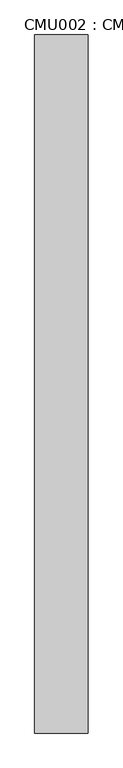
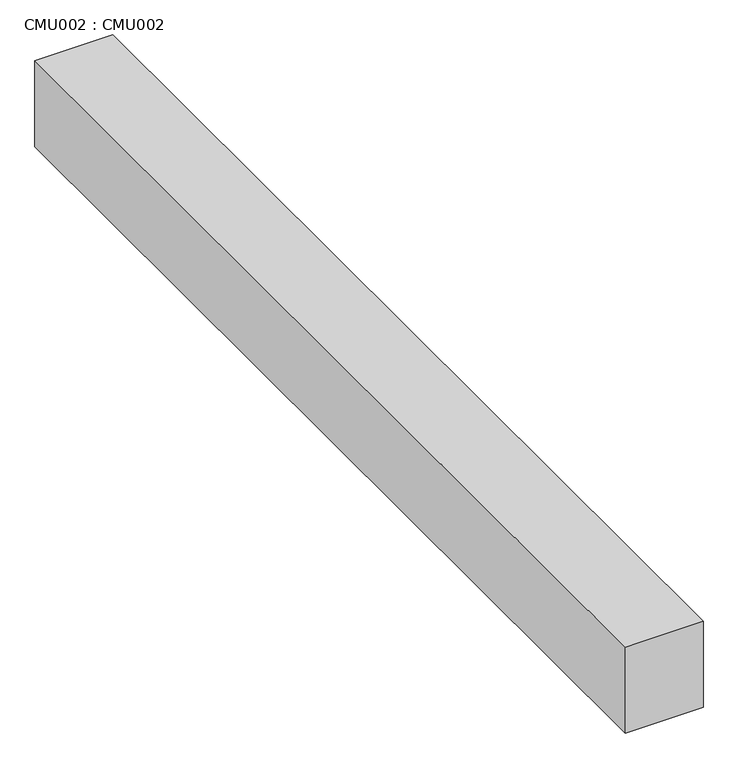
"""IFC4 building model written with IfcOpenShell, lengths in millimetres: proxy geometry, CMU002 : CMU002."""

from ifc_helpers import new_model, si_unit, frame, origin, place, context, project, spatial, polyline, outline, extrude, source, transform, mapped, element, save


def cmu002_cmu002_9a852610(model_context):
    return source(origin(), model_context, "Body", "SweptSolid", [
        extrude(outline(polyline([(-10098.4737014, 7982.1531721), (-10250.8737014, 7982.1531721), (-10250.8737014, 9982.1531721), (-10098.4737014, 9982.1531721), (-10098.4737014, 7982.1531721)])), frame((0.0, 0.0, 32630.4801779), z_axis=(0.0, 0.0, 1.0), x_axis=(1.0, 0.0, 0.0)), (0.0, 0.0, 1.0), 177.8),
    ])


if __name__ == "__main__":
    model = new_model("IFC4")
    model_context = context("Model", 3, world=origin())
    ifc_project = project(units=[si_unit("LENGTHUNIT", "METRE", prefix="MILLI")], contexts=[model_context])
    site = spatial("IfcSite", under=ifc_project)
    building = spatial("IfcBuilding", under=site)
    placement = place(None, origin())
    cmu002_cmu002_shape = cmu002_cmu002_9a852610(model_context)
    element("IfcBuildingElementProxy", 1, Name="CMU002 : CMU002", ObjectType="CMU002 : CMU002", at=placement, inside=building, context=model_context, shape_type="MappedRepresentation", body=[
        mapped(cmu002_cmu002_shape, transform((0.0, 0.0, 0.0), x_axis=(1.0, 0.0, 0.0), y_axis=(0.0, 1.0, 0.0), z_axis=(0.0, 0.0, 1.0))),
    ])
    save(model, "model.ifc")

# Revit data of these elements
# Type "CMU002 : CMU002"
#   NameOverride = "CMU002"
# Element 1 (IfcBuildingElementProxy, "CMU002 : CMU002")
#   Materials on its faces: "4\" CMU WALL"
# Materials
#   "4\" CMU WALL": class "Unassigned", colour RGB 128 128 128, transparency 0, Cost = 0
